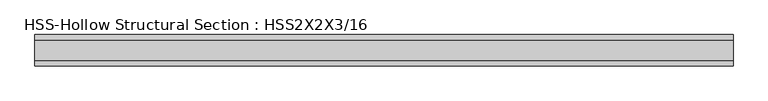
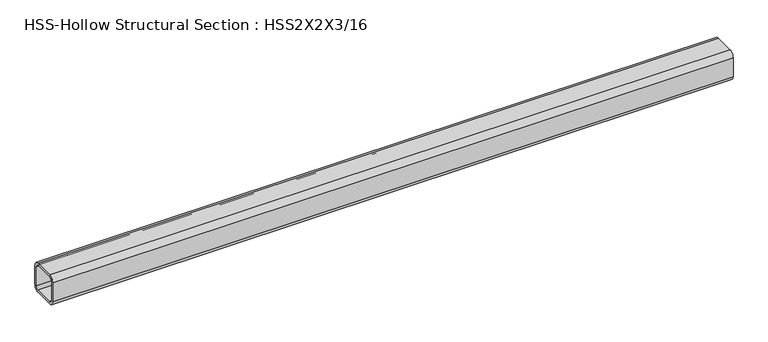
"""IFC4 building model written with IfcOpenShell, lengths in millimetres: beam geometry, HSS-Hollow Structural Section : HSS2X2X3/16."""

from ifc_helpers import new_model, si_unit, point, frame, frame_2d, origin, place, context, project, spatial, polyline, circle_curve, trimmed, segment, composite_curve, outline, extrude, source, transform, mapped, element, save


def hss_hollow_structural_section_hss2x2x3_16_89176741(model_context):
    return source(origin(), model_context, "Body", "SweptSolid", [
        extrude(outline(composite_curve([segment(polyline([(25.4, 16.5608), (25.4, -16.5608)]), True, "CONTINUOUS"), segment(trimmed(circle_curve(frame_2d((16.5608, -16.5608)), 8.8392), [point((25.4, -16.5608))], [point((16.5608, -25.4))], False, "CARTESIAN"), True, "CONTINUOUS"), segment(polyline([(16.5608, -25.4), (-16.5608, -25.4)]), True, "CONTINUOUS"), segment(trimmed(circle_curve(frame_2d((-16.5608, -16.5608)), 8.8392), [point((-16.5608, -25.4))], [point((-25.4, -16.5608))], False, "CARTESIAN"), True, "CONTINUOUS"), segment(polyline([(-25.4, -16.5608), (-25.4, 16.5608)]), True, "CONTINUOUS"), segment(trimmed(circle_curve(frame_2d((-16.5608, 16.5608)), 8.8392), [point((-25.4, 16.5608))], [point((-16.5608, 25.4))], False, "CARTESIAN"), True, "CONTINUOUS"), segment(polyline([(-16.5608, 25.4), (16.5608, 25.4)]), True, "CONTINUOUS"), segment(trimmed(circle_curve(frame_2d((16.5608, 16.5608)), 8.8392), [point((16.5608, 25.4))], [point((25.4, 16.5608))], False, "CARTESIAN"), True, "CONTINUOUS")], self_intersect=False), holes=[composite_curve([segment(trimmed(circle_curve(frame_2d((-16.5608, 16.5608)), 4.4196), [point((-16.5608, 20.9804))], [point((-20.9804, 16.5608))], True, "CARTESIAN"), True, "CONTINUOUS"), segment(polyline([(-20.9804, 16.5608), (-20.9804, -16.5608)]), True, "CONTINUOUS"), segment(trimmed(circle_curve(frame_2d((-16.5608, -16.5608)), 4.4196), [point((-20.9804, -16.5608))], [point((-16.5608, -20.9804))], True, "CARTESIAN"), True, "CONTINUOUS"), segment(polyline([(-16.5608, -20.9804), (16.5608, -20.9804)]), True, "CONTINUOUS"), segment(trimmed(circle_curve(frame_2d((16.5608, -16.5608)), 4.4196), [point((16.5608, -20.9804))], [point((20.9804, -16.5608))], True, "CARTESIAN"), True, "CONTINUOUS"), segment(polyline([(20.9804, -16.5608), (20.9804, 16.5608)]), True, "CONTINUOUS"), segment(trimmed(circle_curve(frame_2d((16.5608, 16.5608)), 4.4196), [point((20.9804, 16.5608))], [point((16.5608, 20.9804))], True, "CARTESIAN"), True, "CONTINUOUS"), segment(polyline([(16.5608, 20.9804), (-16.5608, 20.9804)]), True, "CONTINUOUS")], self_intersect=False)]), frame((8338.34375, 0.0, 0.0), z_axis=(1.0, 0.0, 0.0), x_axis=(0.0, 1.0, 0.0)), (0.0, 0.0, 1.0), 1123.95),
    ])


if __name__ == "__main__":
    model = new_model("IFC4")
    model_context = context("Model", 3, world=origin())
    ifc_project = project(units=[si_unit("LENGTHUNIT", "METRE", prefix="MILLI")], contexts=[model_context])
    site = spatial("IfcSite", under=ifc_project)
    building = spatial("IfcBuilding", under=site)
    placement = place(None, origin())
    hss_hollow_structural_section_hss2x2x3_16_shape = hss_hollow_structural_section_hss2x2x3_16_89176741(model_context)
    element("IfcBeam", 1, ObjectType="HSS-Hollow Structural Section : HSS2X2X3/16", at=placement, inside=building, context=model_context, shape_type="MappedRepresentation", body=[
        mapped(hss_hollow_structural_section_hss2x2x3_16_shape, transform((0.0, 0.0, 0.0), x_axis=(1.0, 0.0, 0.0), y_axis=(0.0, 1.0, 0.0), z_axis=(0.0, 0.0, 1.0))),
    ])
    save(model, "model.ifc")

# Revit data of these elements
# Type "HSS-Hollow Structural Section : HSS2X2X3/16"
#   Keynote = "M05121300.04"
#   Assembly Code = "B10"
#   Shape = "Square"
#   W = 4.3
#   Ht = 0' - 2"
#   Length [instance default] = 5' - 0"
#   b = 0' - 2"
#   kr = 0' - 0.348"
#   t = 0' - 0.174"
#   A = 0.00826389 SF
#   Structural Material [instance default] = Steel ASTM A500, Grade B, Rectangular and Square
# Element 1 (IfcBeam, "HSS-Hollow Structural Section : HSS2X2X3/16")
#   Materials on its faces: "Steel ASTM A500, Grade B, Rectangular and Square"
# Materials
#   "Steel ASTM A500, Grade B, Rectangular and Square": class "Metal", colour RGB 199 199 199, transparency 0, Description = "Carbon steel", Cost = 0
